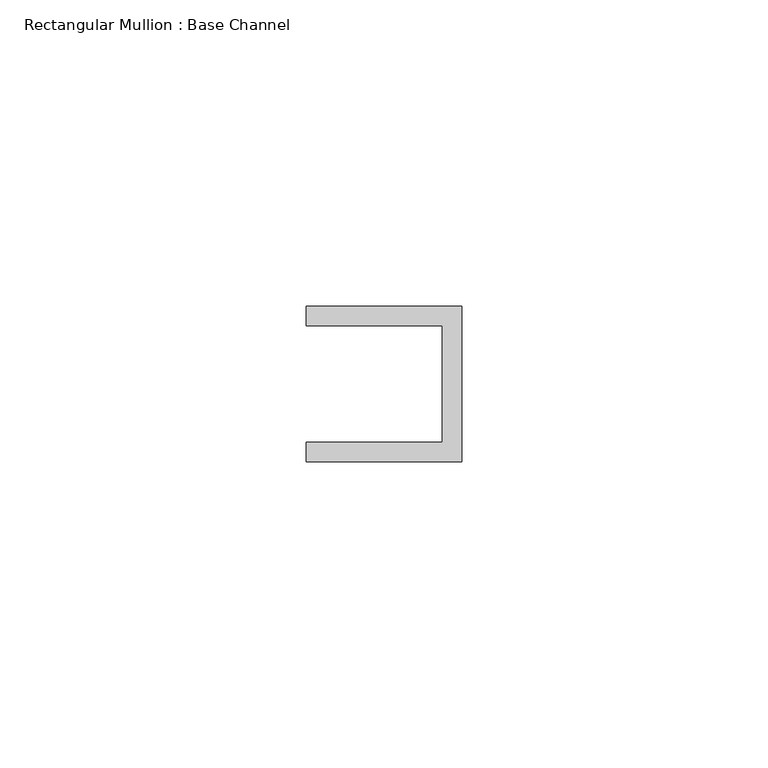
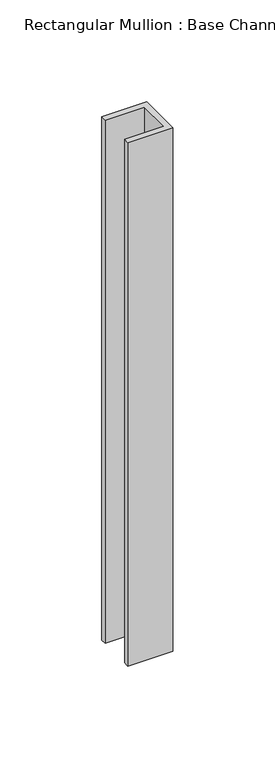
"""IFC4 building model written with IfcOpenShell, lengths in millimetres: member geometry, Rectangular Mullion : Base Channel."""

import ifcopenshell
import ifcopenshell.guid

model = None  # the IFC model being written
_history = None  # IfcOwnerHistory: only IFC2X3 demands one
_inside = {}  # id of a spatial element -> (the spatial element, [elements in it])
_under = {}  # id of a project, library or spatial element -> (it, [spatial elements below it])
_declared = {}  # id of a project -> (the project, [libraries it declares])
_typed = {}  # id of a type object -> (the type object, [elements of that type])
_made_of = {}  # id of a material, layer set ... -> (it, [elements and type objects made of it])


def new_model(schema):
    """Start an empty IFC model of exactly this schema.

    Asked for "IFC4X3", IfcOpenShell would pick the latest addendum, in which some entities
    have other attributes; the version numbers below select the first issue.
    IFC2X3 requires an IfcOwnerHistory on every rooted entity: one is made here for all.
    """
    global model, _history
    if schema == "IFC4X3":
        model = ifcopenshell.file(schema_version=(4, 3, 0, 0))
    else:
        model = ifcopenshell.file(schema=schema)
    _inside.clear()
    _under.clear()
    _declared.clear()
    _typed.clear()
    _made_of.clear()
    _history = None
    if model.schema == "IFC2X3":
        org = make("IfcOrganization", Name="unknown")
        user = make(
            "IfcPersonAndOrganization",
            ThePerson=make("IfcPerson", FamilyName="unknown"),
            TheOrganization=org,
        )
        app = make(
            "IfcApplication",
            ApplicationDeveloper=org,
            Version="unknown",
            ApplicationFullName="unknown",
            ApplicationIdentifier="unknown",
        )
        _history = make(
            "IfcOwnerHistory",
            OwningUser=user,
            OwningApplication=app,
            ChangeAction="ADDED",
            CreationDate=0,
        )
    return model


def make(cls, **values):
    """One entity of the class cls with the attributes given. An attribute that is None is left unset."""
    return model.create_entity(
        cls, **{name: value for name, value in values.items() if value is not None}
    )


def rooted(cls, **values):
    """An entity with a GlobalId (a new one), such as an element, a storey or a relation."""
    return make(cls, GlobalId=ifcopenshell.guid.new(), OwnerHistory=_history, **values)


def si_unit(unit_type, name, prefix=None):
    """IfcSIUnit, for example si_unit("LENGTHUNIT", "METRE", prefix="MILLI")."""
    return make("IfcSIUnit", UnitType=unit_type, Prefix=prefix, Name=name)


def assignment(units):
    """IfcUnitAssignment: the units of a project."""
    return None if units is None else make("IfcUnitAssignment", Units=units)


def point(xyz):
    """IfcCartesianPoint."""
    return None if xyz is None else make("IfcCartesianPoint", Coordinates=xyz)


def direction(xyz):
    """IfcDirection."""
    return None if xyz is None else make("IfcDirection", DirectionRatios=xyz)


def frame(location, z_axis=None, x_axis=None):
    """IfcAxis2Placement3D, a coordinate frame: its origin and axes. An axis left out is left unset."""
    return make(
        "IfcAxis2Placement3D",
        Location=point(location),
        Axis=direction(z_axis),
        RefDirection=direction(x_axis),
    )


def origin():
    """The frame at (0, 0, 0) with its axes left unset."""
    return frame((0.0, 0.0, 0.0))


def place(relative_to, where):
    """IfcLocalPlacement: puts the frame where relative to a parent placement (None: the world)."""
    return make(
        "IfcLocalPlacement", PlacementRelTo=relative_to, RelativePlacement=where
    )


def context(
    kind, dimensions, precision=None, world=None, true_north=None, identifier=None
):
    """IfcGeometricRepresentationContext, for example the 3D "Model" context."""
    return make(
        "IfcGeometricRepresentationContext",
        ContextIdentifier=identifier,
        ContextType=kind,
        CoordinateSpaceDimension=dimensions,
        Precision=precision,
        WorldCoordinateSystem=world,
        TrueNorth=true_north,
    )


def project(units=None, contexts=None):
    """IfcProject with its units and contexts."""
    return rooted(
        "IfcProject",
        Name="project",
        RepresentationContexts=contexts,
        UnitsInContext=assignment(units),
    )


def spatial(cls, under=None, at=None, **own):
    """A site, building, storey or space (cls), placed at a placement, below another one or the project."""
    s = rooted(cls, ObjectPlacement=at, **own)
    if under is not None:
        _under.setdefault(under.id(), (under, []))[1].append(s)
    return s


def polyline(points):
    """IfcPolyline through the points."""
    return make("IfcPolyline", Points=[point(p) for p in points])


def outline(outer, holes=None, kind="AREA"):
    """IfcArbitraryClosedProfileDef: a profile drawn as a closed curve; with holes, ...WithVoids."""
    if holes is None:
        return make("IfcArbitraryClosedProfileDef", ProfileType=kind, OuterCurve=outer)
    return make(
        "IfcArbitraryProfileDefWithVoids",
        ProfileType=kind,
        OuterCurve=outer,
        InnerCurves=holes,
    )


def extrude(swept, where, along, depth):
    """IfcExtrudedAreaSolid: the profile swept, set in the frame where, extruded along a direction by depth."""
    return make(
        "IfcExtrudedAreaSolid",
        SweptArea=swept,
        Position=where,
        ExtrudedDirection=direction(along),
        Depth=depth,
    )


def shape(context_of_items, identifier, shape_type, items):
    """IfcShapeRepresentation: the items that make up one representation, for example the "Body"."""
    return make(
        "IfcShapeRepresentation",
        ContextOfItems=context_of_items,
        RepresentationIdentifier=identifier,
        RepresentationType=shape_type,
        Items=items,
    )


def source(mapping_origin, context_of_items, identifier, shape_type, items):
    """IfcRepresentationMap: a shape defined once, which mapped items show again and again."""
    return make(
        "IfcRepresentationMap",
        MappingOrigin=mapping_origin,
        MappedRepresentation=shape(context_of_items, identifier, shape_type, items),
    )


def transform(
    local_origin,
    x_axis=None,
    y_axis=None,
    z_axis=None,
    scale=None,
    scale2=None,
    scale3=None,
    uniform=True,
):
    """IfcCartesianTransformationOperator3D, or its non-uniform kind. x_axis, y_axis, z_axis: its Axis1, 2, 3."""
    if uniform:
        return make(
            "IfcCartesianTransformationOperator3D",
            Axis1=direction(x_axis),
            Axis2=direction(y_axis),
            LocalOrigin=point(local_origin),
            Scale=scale,
            Axis3=direction(z_axis),
        )
    return make(
        "IfcCartesianTransformationOperator3DnonUniform",
        Axis1=direction(x_axis),
        Axis2=direction(y_axis),
        LocalOrigin=point(local_origin),
        Scale=scale,
        Axis3=direction(z_axis),
        Scale2=scale2,
        Scale3=scale3,
    )


def mapped(mapping_source, mapping_target):
    """IfcMappedItem: shows the shape of a source again, moved by a transform."""
    return make(
        "IfcMappedItem", MappingSource=mapping_source, MappingTarget=mapping_target
    )


def made_of(thing, what):
    """Note that an element or type object is made of a material, layer set ...; save() writes the relation."""
    if what is not None:
        _made_of.setdefault(what.id(), (what, []))[1].append(thing)
    return thing


def element(
    cls,
    number,
    at=None,
    inside=None,
    cuts=None,
    type_object=None,
    material=None,
    context=None,
    identifier="Body",
    shape_type=None,
    held_by="IfcProductDefinitionShape",
    body=None,
    shapes=None,
    **own,
):
    """One element of the class cls, such as IfcWall. Its Tag is "e" and its number.

    at: its placement. inside: the storey or other place that contains it. cuts: it is an
    opening in that element (IfcRelVoidsElement). A single representation is given by context,
    identifier, shape_type and body (its items); several are given by shapes. held_by: the class
    of the entity that holds the representations. save() writes the other relations.
    """
    e = rooted(cls, Tag="e%d" % number, ObjectPlacement=at, **own)
    if body is not None:
        shapes = [shape(context, identifier, shape_type, body)]
    if shapes is not None:
        e.Representation = make(held_by, Representations=shapes)
    if inside is not None:
        _inside.setdefault(inside.id(), (inside, []))[1].append(e)
    if cuts is not None:
        rooted(
            "IfcRelVoidsElement", RelatingBuildingElement=cuts, RelatedOpeningElement=e
        )
    if type_object is not None:
        _typed.setdefault(type_object.id(), (type_object, []))[1].append(e)
    return made_of(e, material)


def aggregate(whole, parts):
    """IfcRelAggregates: a whole, such as a stair, and the parts it consists of."""
    return rooted("IfcRelAggregates", RelatingObject=whole, RelatedObjects=parts)


def save(model, path):
    """Write the relations noted so far, then the file.

    IfcRelAggregates (storeys below a building ...), IfcRelContainedInSpatialStructure (elements
    in a storey), IfcRelDefinesByType, IfcRelAssociatesMaterial and IfcRelDeclares: one each for
    every whole, place, type object, material and project.
    """
    for whole, parts in _under.values():
        aggregate(whole, parts)
    for where, things in _inside.values():
        rooted(
            "IfcRelContainedInSpatialStructure",
            RelatedElements=things,
            RelatingStructure=where,
        )
    for kind, things in _typed.values():
        rooted("IfcRelDefinesByType", RelatedObjects=things, RelatingType=kind)
    for what, things in _made_of.values():
        rooted("IfcRelAssociatesMaterial", RelatedObjects=things, RelatingMaterial=what)
    for by, libraries in _declared.values():
        rooted("IfcRelDeclares", RelatingContext=by, RelatedDefinitions=libraries)
    model.write(path)


def rectangular_mullion_base_channel_d4df9a30(model_context):
    return source(origin(), model_context, "Body", "SweptSolid", [
        extrude(outline(polyline([(0.0, -12.7), (-25.4, -12.7), (-25.4, -9.525), (-3.175, -9.525), (-3.175, 9.525), (-25.4, 9.525), (-25.4, 12.7), (0.0, 12.7), (0.0, -12.7)])), frame((0.0, 0.0, -313.2666667), z_axis=(0.0, 0.0, 1.0), x_axis=(1.0, 0.0, 0.0)), (0.0, 0.0, 1.0), 313.2666667),
    ])


if __name__ == "__main__":
    model = new_model("IFC4")
    model_context = context("Model", 3, world=origin())
    ifc_project = project(units=[si_unit("LENGTHUNIT", "METRE", prefix="MILLI")], contexts=[model_context])
    site = spatial("IfcSite", under=ifc_project)
    building = spatial("IfcBuilding", under=site)
    placement = place(None, origin())
    rectangular_mullion_base_channel_shape = rectangular_mullion_base_channel_d4df9a30(model_context)
    element("IfcMember", 1, ObjectType="Rectangular Mullion : Base Channel", at=placement, inside=building, context=model_context, shape_type="MappedRepresentation", body=[
        mapped(rectangular_mullion_base_channel_shape, transform((0.0, 0.0, 0.0), x_axis=(1.0, 0.0, 0.0), y_axis=(0.0, 1.0, 0.0), z_axis=(0.0, 0.0, 1.0))),
    ])
    save(model, "model.ifc")

# Revit data of these elements
# Type "Rectangular Mullion : Base Channel"
#   built-in parameter 1007322 = 0.0833333 (stored number, unit not read)
#   built-in parameter 1007321 = 0.0416667 (stored number, unit not read)
#   built-in parameter 1007320 = -0.03125 (stored number, unit not read)
# Element 1 (IfcMember, "Rectangular Mullion : Base Channel")
#   Materials on its faces: "ALUM"
# Materials
#   "ALUM": class "Generic", colour RGB 157 157 157, transparency 0, Cost = 0
